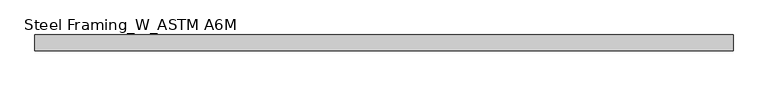
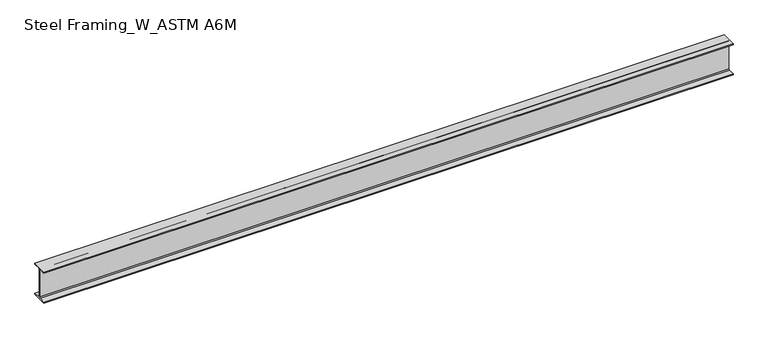
"""IFC4 building model written with IfcOpenShell, lengths in millimetres: beam geometry, Steel Framing_W_ASTM A6M : H_SB_AR_S02_W360x51_G3."""

from ifc_helpers import new_model, si_unit, point, frame, frame_2d, origin, place, context, project, spatial, polyline, circle_curve, trimmed, segment, composite_curve, outline, extrude, source, transform, mapped, element, save


def steel_framing_w_astm_a6m_c8f375b8(model_context):
    return source(origin(), model_context, "Body", "SweptSolid", [
        extrude(outline(composite_curve([segment(polyline([(85.5, -166.4), (85.5, -178.0), (-85.5, -178.0), (-85.5, -166.4), (-13.72, -166.4)]), True, "CONTINUOUS"), segment(trimmed(circle_curve(frame_2d((-13.72, -156.3)), 10.1), [point((-13.72, -166.4))], [point((-3.62, -156.3))], True, "CARTESIAN"), True, "CONTINUOUS"), segment(polyline([(-3.62, -156.3), (-3.62, 156.3)]), True, "CONTINUOUS"), segment(trimmed(circle_curve(frame_2d((-13.72, 156.3)), 10.1), [point((-3.62, 156.3))], [point((-13.72, 166.4))], True, "CARTESIAN"), True, "CONTINUOUS"), segment(polyline([(-13.72, 166.4), (-85.5, 166.4), (-85.5, 178.0), (85.5, 178.0), (85.5, 166.4), (13.72, 166.4)]), True, "CONTINUOUS"), segment(trimmed(circle_curve(frame_2d((13.72, 156.3)), 10.1), [point((13.72, 166.4))], [point((3.62, 156.3))], True, "CARTESIAN"), True, "CONTINUOUS"), segment(polyline([(3.62, 156.3), (3.62, -156.3)]), True, "CONTINUOUS"), segment(trimmed(circle_curve(frame_2d((13.72, -156.3)), 10.1), [point((3.62, -156.3))], [point((13.72, -166.4))], True, "CARTESIAN"), True, "CONTINUOUS"), segment(polyline([(13.72, -166.4), (85.5, -166.4)]), True, "CONTINUOUS")], self_intersect=False)), frame((-3753.7, 0.0, 0.0), z_axis=(1.0, 0.0, 0.0), x_axis=(0.0, 1.0, 0.0)), (0.0, 0.0, 1.0), 7507.4),
    ])


if __name__ == "__main__":
    model = new_model("IFC4")
    model_context = context("Model", 3, world=origin())
    ifc_project = project(units=[si_unit("LENGTHUNIT", "METRE", prefix="MILLI")], contexts=[model_context])
    site = spatial("IfcSite", under=ifc_project)
    building = spatial("IfcBuilding", under=site)
    placement = place(None, origin())
    steel_framing_w_astm_a6m_shape = steel_framing_w_astm_a6m_c8f375b8(model_context)
    element("IfcBeam", 1, ObjectType="Steel Framing_W_ASTM A6M : H_SB_AR_S02_W360x51_G3", at=placement, inside=building, context=model_context, shape_type="MappedRepresentation", body=[
        mapped(steel_framing_w_astm_a6m_shape, transform((0.0, 0.0, 0.0), x_axis=(1.0, 0.0, 0.0), y_axis=(0.0, 1.0, 0.0), z_axis=(0.0, 0.0, 1.0))),
    ])
    save(model, "model.ifc")

# Revit data of these elements
# Type "Steel Framing_W_ASTM A6M : H_SB_AR_S02_W360x51_G3"
#   Type Mark = "G3"
#   Section Name Key = "W14x34"
#   Width = 17.1 cm
#   Web Thickness = 0.724 cm
#   Web Fillet = 1.01 cm
#   Warping Constant = 287000.0 cm⁶
#   Torsional Moment of Inertia = 23.70 cm⁴
#   Section Area = 64.5 cm²
#   Plastic Modulus weak axis = 174.0 cm³
#   Plastic Modulus strong axis = 895.0 cm³
#   Perimeter = 1.36 m²/m
#   Nominal Weight = 51.00 kgf/m
#   Moment of Inertia weak axis = 970.00 cm⁴
#   Moment of Inertia strong axis = 14200.00 cm⁴
#   Height = 35.6 cm
#   Flange Thickness = 1.16 cm
#   Elastic Modulus weak axis = 113.0 cm³
#   Elastic Modulus strong axis = 796.0 cm³
#   Centroid Vertical = 17.8 cm
#   Centroid Horizontal = 8.55 cm
#   Length [instance default] = 1500 mm
#   Structural Material [instance default] = Steel, 45-345
#   Bolt Spacing = 0
#   Assembly Code = ""
# Element 1 (IfcBeam, "Steel Framing_W_ASTM A6M : H_SB_AR_S02_W360x51_G3")
#   Materials on its faces: "Steel, 45-345"
# Materials
#   "Steel, 45-345": class "Metal", colour RGB 189 187 185, transparency 0, Description = "Steel 345 MPa", Cost = 0
